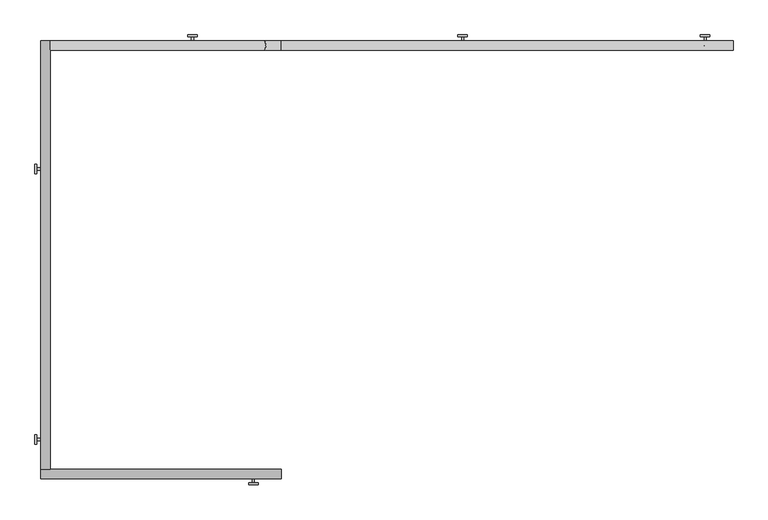
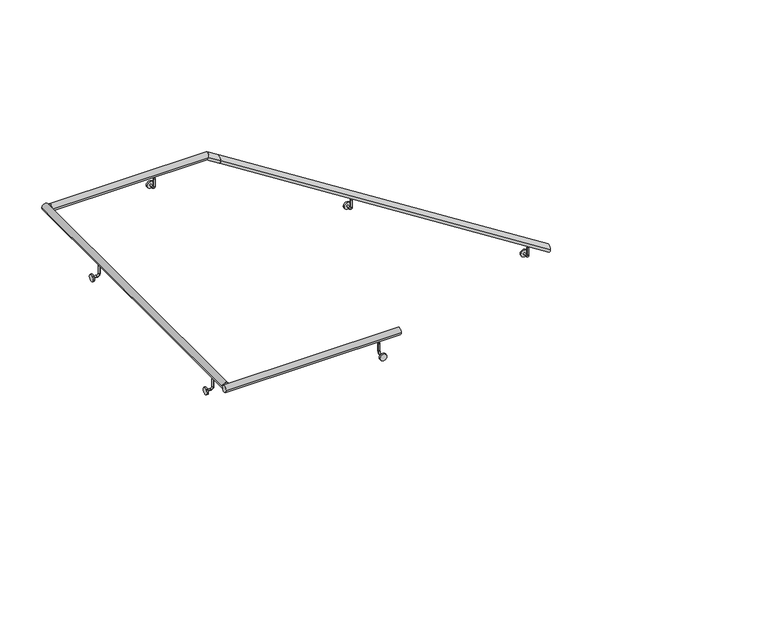
"""IFC4 building model written with IfcOpenShell, lengths in millimetres: railing geometry."""

from ifc_helpers import new_model, si_unit, point, frame, frame_2d, origin, place, context, project, spatial, circle_curve, ellipse_curve, trimmed, segment, composite_curve, outline, extrude, source, transform, mapped, element, save
from ifc_brep_helpers import plane_surface, cylinder_surface, revolved_surface, advanced_brep


def railing_d584f0b8(model_context):
    return source(origin(), model_context, "Body", "SolidModel", [
        advanced_brep(
        [(-47747.4858495, 17739.1574868, 4652.1467196), (-47747.4858495, 17789.1574868, 4652.1467196), (-50177.4858495, 17739.1574868, 6195.0038624), (-50177.4858495, 17789.1574868, 6195.0038624)],
        [
            (0, 1, ellipse_curve(frame((-47747.4858495, 17764.1574868, 4652.1467196), z_axis=(1.0, 0.0, 0.0), x_axis=(0.0, 0.0, -1.0)), 29.613386, 25.0)),
            (1, 0, ellipse_curve(frame((-47747.4858495, 17764.1574868, 4652.1467196), z_axis=(1.0, 0.0, 0.0), x_axis=(0.0, 0.0, -1.0)), 29.613386, 25.0)),
            (2, 3, ellipse_curve(frame((-50177.4858495, 17764.1574868, 6195.0038624), z_axis=(-1.0, 0.0, 0.0), x_axis=(0.0, 0.0, -1.0)), 29.613386, 25.0)),
            (3, 2, ellipse_curve(frame((-50177.4858495, 17764.1574868, 6195.0038624), z_axis=(-1.0, 0.0, 0.0), x_axis=(0.0, 0.0, -1.0)), 29.613386, 25.0)),
            (0, 2),
            (3, 1),
        ],
        [
            plane_surface(frame((-47747.4858495, 17764.1574868, 4681.7601056), z_axis=(1.0, 0.0, 0.0), x_axis=(0.0, -1.0, 0.0))),
            plane_surface(frame((-50177.4858495, 17764.1574868, 6224.6172485), z_axis=(-1.0, 0.0, 0.0), x_axis=(0.0, -1.0, 0.0))),
            cylinder_surface(frame((-47760.8860529, 17764.1574868, 4660.6547852), z_axis=(0.8442128152478047, 0.0, -0.5360081366652713), x_axis=(0.0, 1.0, 0.0)), 25.0),
        ],
        [
            (0, [[1, 2]]),
            (1, [[3, 4]]),
            (2, [[-1, 5, -4, 6]]),
            (2, [[-2, -6, -3, -5]]),
        ],
    ),
        advanced_brep(
        [(-50177.4858495, 17739.1574868, 6195.0038624), (-50177.4858495, 17789.1574868, 6195.0038624), (-50268.4797662, 17739.1574868, 6252.7777778), (-50268.4797662, 17789.1574868, 6252.7777778), (-51419.7848926, 17739.1574868, 6252.7777778), (-51419.7848926, 17789.1574868, 6252.7777778)],
        [
            (0, 1, ellipse_curve(frame((-50177.4858495, 17764.1574868, 6195.0038624), z_axis=(1.0, 0.0, 0.0), x_axis=(0.0, 0.0, -1.0)), 29.613386, 25.0)),
            (1, 0, ellipse_curve(frame((-50177.4858495, 17764.1574868, 6195.0038624), z_axis=(1.0, 0.0, 0.0), x_axis=(0.0, 0.0, -1.0)), 29.613386, 25.0)),
            (0, 2),
            (2, 3, ellipse_curve(frame((-50268.4797662, 17764.1574868, 6252.7777778), z_axis=(0.9602637177483601, 0.0, -0.27909423565544655), x_axis=(-0.2790942356554468, 0.0, -0.9602637177483601)), 26.0345148, 25.0)),
            (3, 1),
            (3, 2, ellipse_curve(frame((-50268.4797662, 17764.1574868, 6252.7777778), z_axis=(0.9602637177483601, 0.0, -0.27909423565544655), x_axis=(-0.2790942356554468, 0.0, -0.9602637177483601)), 26.0345148, 25.0)),
            (4, 5, circle_curve(frame((-51419.7848926, 17764.1574868, 6252.7777778), z_axis=(-1.0, 0.0, 0.0), x_axis=(0.0, 1.0, 0.0)), 25.0)),
            (5, 4, circle_curve(frame((-51419.7848926, 17764.1574868, 6252.7777778), z_axis=(-1.0, 0.0, 0.0), x_axis=(0.0, 1.0, 0.0)), 25.0)),
            (2, 4),
            (5, 3),
        ],
        [
            plane_surface(frame((-50177.4858495, 17764.1574868, 6224.6172485), z_axis=(1.0, 0.0, 0.0), x_axis=(0.0, -1.0, 0.0))),
            cylinder_surface(frame((-50190.8860529, 17764.1574868, 6203.5119281), z_axis=(0.844212815247804, 0.0, -0.5360081366652723), x_axis=(0.0, 1.0, 0.0)), 25.0),
            plane_surface(frame((-51419.7848926, 17764.1574868, 6277.7777778), z_axis=(-1.0, 0.0, 0.0), x_axis=(0.0, -1.0, 0.0))),
            cylinder_surface(frame((-50261.2136831, 17764.1574868, 6252.7777778), z_axis=(1.0, 0.0, 0.0), x_axis=(0.0, 1.0, 0.0)), 25.0),
        ],
        [
            (0, [[1, 2]]),
            (1, [[-1, 3, 4, 5]]),
            (1, [[-2, -5, 6, -3]]),
            (2, [[7, 8]]),
            (3, [[-4, 9, -8, 10]]),
            (3, [[-6, -10, -7, -9]]),
        ],
    ),
        advanced_brep(
        [(-51419.7848926, 17789.1574868, 6252.7777778), (-51469.7848926, 17789.1574868, 6252.7777778), (-51419.7848926, 15484.3574868, 6252.7777778), (-51469.7848926, 15484.3574868, 6252.7777778)],
        [
            (0, 1, circle_curve(frame((-51444.7848926, 17789.1574868, 6252.7777778), z_axis=(0.0, 1.0, 0.0), x_axis=(-1.0, 0.0, 0.0)), 25.0)),
            (1, 0, circle_curve(frame((-51444.7848926, 17789.1574868, 6252.7777778), z_axis=(0.0, 1.0, 0.0), x_axis=(-1.0, 0.0, 0.0)), 25.0)),
            (2, 3, circle_curve(frame((-51444.7848926, 15484.3574868, 6252.7777778), z_axis=(0.0, -1.0, 0.0), x_axis=(-1.0, 0.0, 0.0)), 25.0)),
            (3, 2, circle_curve(frame((-51444.7848926, 15484.3574868, 6252.7777778), z_axis=(0.0, -1.0, 0.0), x_axis=(-1.0, 0.0, 0.0)), 25.0)),
            (0, 2),
            (3, 1),
        ],
        [
            plane_surface(frame((-51444.7848926, 17789.1574868, 6277.7777778), z_axis=(0.0, 1.0, 0.0), x_axis=(0.0, 0.0, -1.0))),
            plane_surface(frame((-51444.7848926, 15484.3574868, 6277.7777778), z_axis=(0.0, -1.0, 0.0), x_axis=(0.0, 0.0, -1.0))),
            cylinder_surface(frame((-51444.7848926, 17789.1574868, 6252.7777778), z_axis=(0.0, 1.0, 0.0), x_axis=(-1.0, 0.0, 0.0)), 25.0),
        ],
        [
            (0, [[1, 2]]),
            (1, [[3, 4]]),
            (2, [[-1, 5, -4, 6]]),
            (2, [[-2, -6, -3, -5]]),
        ],
    ),
        advanced_brep(
        [(-51469.7848926, 15484.3574868, 6252.7777778), (-51469.7848926, 15434.3574868, 6252.7777778), (-50177.4858495, 15484.3574868, 6252.7777778), (-50177.4858495, 15434.3574868, 6252.7777778)],
        [
            (0, 1, circle_curve(frame((-51469.7848926, 15459.3574868, 6252.7777778), z_axis=(-1.0, 0.0, 0.0), x_axis=(0.0, -1.0, 0.0)), 25.0)),
            (1, 0, circle_curve(frame((-51469.7848926, 15459.3574868, 6252.7777778), z_axis=(-1.0, 0.0, 0.0), x_axis=(0.0, -1.0, 0.0)), 25.0)),
            (2, 3, circle_curve(frame((-50177.4858495, 15459.3574868, 6252.7777778), z_axis=(1.0, 0.0, 0.0), x_axis=(0.0, -1.0, 0.0)), 25.0)),
            (3, 2, circle_curve(frame((-50177.4858495, 15459.3574868, 6252.7777778), z_axis=(1.0, 0.0, 0.0), x_axis=(0.0, -1.0, 0.0)), 25.0)),
            (0, 2),
            (3, 1),
        ],
        [
            plane_surface(frame((-51469.7848926, 15459.3574868, 6277.7777778), z_axis=(-1.0, 0.0, 0.0), x_axis=(0.0, 1.0, 0.0))),
            plane_surface(frame((-50177.4858495, 15459.3574868, 6277.7777778), z_axis=(1.0, 0.0, 0.0), x_axis=(0.0, 1.0, 0.0))),
            cylinder_surface(frame((-51469.7848926, 15459.3574868, 6252.7777778), z_axis=(-1.0, 0.0, 0.0), x_axis=(0.0, -1.0, 0.0)), 25.0),
        ],
        [
            (0, [[1, 2]]),
            (1, [[3, 4]]),
            (2, [[-1, 5, -4, 6]]),
            (2, [[-2, -6, -3, -5]]),
        ],
    ),
        advanced_brep(
        [(-51444.7848926, 15652.288061, 6208.7277778), (-51444.7848926, 15639.588061, 6208.7277778), (-51444.7848926, 15652.288061, 6151.5777778), (-51444.7848926, 15639.588061, 6151.5777778), (-51463.8348926, 15639.588061, 6132.5277778), (-51463.8348926, 15652.288061, 6132.5277778), (-51492.4098926, 15652.288061, 6132.5277778), (-51492.4098926, 15639.588061, 6132.5277778)],
        [
            (0, 1, circle_curve(frame((-51444.7848926, 15645.938061, 6208.7277778), z_axis=(0.0, 0.0, 1.0), x_axis=(0.0, -1.0, 0.0)), 6.35)),
            (1, 0, circle_curve(frame((-51444.7848926, 15645.938061, 6208.7277778), z_axis=(0.0, 0.0, 1.0), x_axis=(0.0, -1.0, 0.0)), 6.35)),
            (0, 2),
            (2, 3, circle_curve(frame((-51444.7848926, 15645.938061, 6151.5777778), z_axis=(0.0, 0.0, 1.0), x_axis=(0.0, -1.0, 0.0)), 6.35)),
            (3, 1),
            (3, 2, circle_curve(frame((-51444.7848926, 15645.938061, 6151.5777778), z_axis=(0.0, 0.0, 1.0), x_axis=(0.0, -1.0, 0.0)), 6.35)),
            (4, 3, circle_curve(frame((-51463.8348926, 15639.588061, 6151.5777778), z_axis=(0.0, -1.0, 0.0), x_axis=(1.0, 0.0, 0.0)), 19.05)),
            (2, 5, circle_curve(frame((-51463.8348926, 15652.288061, 6151.5777778), z_axis=(0.0, 1.0, 0.0), x_axis=(1.0, 0.0, 0.0)), 19.05)),
            (5, 4, circle_curve(frame((-51463.8348926, 15645.938061, 6132.5277778), z_axis=(1.0, 0.0, 0.0), x_axis=(0.0, -1.0, 0.0)), 6.35)),
            (4, 5, circle_curve(frame((-51463.8348926, 15645.938061, 6132.5277778), z_axis=(1.0, 0.0, 0.0), x_axis=(0.0, -1.0, 0.0)), 6.35)),
            (6, 7, circle_curve(frame((-51492.4098926, 15645.938061, 6132.5277778), z_axis=(-1.0, 0.0, 0.0), x_axis=(0.0, -1.0, 0.0)), 6.35)),
            (7, 6, circle_curve(frame((-51492.4098926, 15645.938061, 6132.5277778), z_axis=(-1.0, 0.0, 0.0), x_axis=(0.0, -1.0, 0.0)), 6.35)),
            (5, 6),
            (7, 4),
        ],
        [
            plane_surface(frame((-51444.7848926, 15639.588061, 6208.7277778), z_axis=(0.0, 0.0, 1.0), x_axis=(-1.0, 0.0, 0.0))),
            cylinder_surface(frame((-51444.7848926, 15645.938061, 6208.7277778), z_axis=(0.0, 0.0, 1.0), x_axis=(0.0, -1.0, 0.0)), 6.35),
            revolved_surface(trimmed(ellipse_curve(frame((-51444.7848926, 15645.938061, 6151.5777778), z_axis=(0.0, 0.0, 1.0), x_axis=(0.0, -1.0, 0.0)), 6.35, 6.35), [point((-51444.7848926, 15652.288061, 6151.5777778))], [point((-51444.7848926, 15639.588061, 6151.5777778))], True, "CARTESIAN"), (-51463.8348926, 15645.938061, 6151.5777778), (0.0, 1.0, 0.0)),
            revolved_surface(trimmed(ellipse_curve(frame((-51444.7848926, 15645.938061, 6151.5777778), z_axis=(0.0, 0.0, 1.0), x_axis=(0.0, -1.0, 0.0)), 6.35, 6.35), [point((-51444.7848926, 15639.588061, 6151.5777778))], [point((-51444.7848926, 15652.288061, 6151.5777778))], True, "CARTESIAN"), (-51463.8348926, 15645.938061, 6151.5777778), (0.0, 1.0, 0.0)),
            plane_surface(frame((-51492.4098926, 15645.938061, 6126.1777778), z_axis=(-1.0, 0.0, 0.0), x_axis=(0.0, -1.0, 0.0))),
            cylinder_surface(frame((-51463.8348926, 15645.938061, 6132.5277778), z_axis=(1.0, 0.0, 0.0), x_axis=(0.0, -1.0, 0.0)), 6.35),
        ],
        [
            (0, [[1, 2]]),
            (1, [[-1, 3, 4, 5]]),
            (1, [[-2, -5, 6, -3]]),
            (2, [[7, -4, 8, 9]]),
            (3, [[-8, -6, -7, 10]]),
            (4, [[11, 12]]),
            (5, [[-9, 13, -12, 14]]),
            (5, [[-10, -14, -11, -13]]),
        ],
    ),
        extrude(outline(composite_curve([segment(trimmed(circle_curve(frame_2d((15645.938061, 6132.5277778)), 25.4), [point((15620.538061, 6132.5277778))], [point((15671.338061, 6132.5277778))], False, "CARTESIAN"), True, "CONTINUOUS"), segment(trimmed(circle_curve(frame_2d((15645.938061, 6132.5277778)), 25.4), [point((15671.338061, 6132.5277778))], [point((15620.538061, 6132.5277778))], False, "CARTESIAN"), True, "CONTINUOUS")], self_intersect=False)), frame((-51501.9348926, 0.0, 0.0), z_axis=(1.0, 0.0, 0.0), x_axis=(0.0, 1.0, 0.0)), (0.0, 0.0, 1.0), 9.525),
        advanced_brep(
        [(-51444.7848926, 17106.1676782, 6208.7277778), (-51444.7848926, 17093.4676782, 6208.7277778), (-51444.7848926, 17106.1676782, 6151.5777778), (-51444.7848926, 17093.4676782, 6151.5777778), (-51463.8348926, 17093.4676782, 6132.5277778), (-51463.8348926, 17106.1676782, 6132.5277778), (-51492.4098926, 17106.1676782, 6132.5277778), (-51492.4098926, 17093.4676782, 6132.5277778)],
        [
            (0, 1, circle_curve(frame((-51444.7848926, 17099.8176782, 6208.7277778), z_axis=(0.0, 0.0, 1.0), x_axis=(0.0, -1.0, 0.0)), 6.35)),
            (1, 0, circle_curve(frame((-51444.7848926, 17099.8176782, 6208.7277778), z_axis=(0.0, 0.0, 1.0), x_axis=(0.0, -1.0, 0.0)), 6.35)),
            (0, 2),
            (2, 3, circle_curve(frame((-51444.7848926, 17099.8176782, 6151.5777778), z_axis=(0.0, 0.0, 1.0), x_axis=(0.0, -1.0, 0.0)), 6.35)),
            (3, 1),
            (3, 2, circle_curve(frame((-51444.7848926, 17099.8176782, 6151.5777778), z_axis=(0.0, 0.0, 1.0), x_axis=(0.0, -1.0, 0.0)), 6.35)),
            (4, 3, circle_curve(frame((-51463.8348926, 17093.4676782, 6151.5777778), z_axis=(0.0, -1.0, 0.0), x_axis=(1.0, 0.0, 0.0)), 19.05)),
            (2, 5, circle_curve(frame((-51463.8348926, 17106.1676782, 6151.5777778), z_axis=(0.0, 1.0, 0.0), x_axis=(1.0, 0.0, 0.0)), 19.05)),
            (5, 4, circle_curve(frame((-51463.8348926, 17099.8176782, 6132.5277778), z_axis=(1.0, 0.0, 0.0), x_axis=(0.0, -1.0, 0.0)), 6.35)),
            (4, 5, circle_curve(frame((-51463.8348926, 17099.8176782, 6132.5277778), z_axis=(1.0, 0.0, 0.0), x_axis=(0.0, -1.0, 0.0)), 6.35)),
            (6, 7, circle_curve(frame((-51492.4098926, 17099.8176782, 6132.5277778), z_axis=(-1.0, 0.0, 0.0), x_axis=(0.0, -1.0, 0.0)), 6.35)),
            (7, 6, circle_curve(frame((-51492.4098926, 17099.8176782, 6132.5277778), z_axis=(-1.0, 0.0, 0.0), x_axis=(0.0, -1.0, 0.0)), 6.35)),
            (5, 6),
            (7, 4),
        ],
        [
            plane_surface(frame((-51444.7848926, 17093.4676782, 6208.7277778), z_axis=(0.0, 0.0, 1.0), x_axis=(-1.0, 0.0, 0.0))),
            cylinder_surface(frame((-51444.7848926, 17099.8176782, 6208.7277778), z_axis=(0.0, 0.0, 1.0), x_axis=(0.0, -1.0, 0.0)), 6.35),
            revolved_surface(trimmed(ellipse_curve(frame((-51444.7848926, 17099.8176782, 6151.5777778), z_axis=(0.0, 0.0, 1.0), x_axis=(0.0, -1.0, 0.0)), 6.35, 6.35), [point((-51444.7848926, 17106.1676782, 6151.5777778))], [point((-51444.7848926, 17093.4676782, 6151.5777778))], True, "CARTESIAN"), (-51463.8348926, 17099.8176782, 6151.5777778), (0.0, 1.0, 0.0)),
            revolved_surface(trimmed(ellipse_curve(frame((-51444.7848926, 17099.8176782, 6151.5777778), z_axis=(0.0, 0.0, 1.0), x_axis=(0.0, -1.0, 0.0)), 6.35, 6.35), [point((-51444.7848926, 17093.4676782, 6151.5777778))], [point((-51444.7848926, 17106.1676782, 6151.5777778))], True, "CARTESIAN"), (-51463.8348926, 17099.8176782, 6151.5777778), (0.0, 1.0, 0.0)),
            plane_surface(frame((-51492.4098926, 17099.8176782, 6126.1777778), z_axis=(-1.0, 0.0, 0.0), x_axis=(0.0, -1.0, 0.0))),
            cylinder_surface(frame((-51463.8348926, 17099.8176782, 6132.5277778), z_axis=(1.0, 0.0, 0.0), x_axis=(0.0, -1.0, 0.0)), 6.35),
        ],
        [
            (0, [[1, 2]]),
            (1, [[-1, 3, 4, 5]]),
            (1, [[-2, -5, 6, -3]]),
            (2, [[7, -4, 8, 9]]),
            (3, [[-8, -6, -7, 10]]),
            (4, [[11, 12]]),
            (5, [[-9, 13, -12, 14]]),
            (5, [[-10, -14, -11, -13]]),
        ],
    ),
        extrude(outline(composite_curve([segment(trimmed(circle_curve(frame_2d((17099.8176782, 6132.5277778)), 25.4), [point((17074.4176782, 6132.5277778))], [point((17125.2176782, 6132.5277778))], False, "CARTESIAN"), True, "CONTINUOUS"), segment(trimmed(circle_curve(frame_2d((17099.8176782, 6132.5277778)), 25.4), [point((17125.2176782, 6132.5277778))], [point((17074.4176782, 6132.5277778))], False, "CARTESIAN"), True, "CONTINUOUS")], self_intersect=False)), frame((-51501.9348926, 0.0, 0.0), z_axis=(1.0, 0.0, 0.0), x_axis=(0.0, 1.0, 0.0)), (0.0, 0.0, 1.0), 9.525),
        advanced_brep(
        [(-50648.895084, 17764.1574868, 6208.7277778), (-50661.595084, 17764.1574868, 6208.7277778), (-50648.895084, 17764.1574868, 6151.5777778), (-50661.595084, 17764.1574868, 6151.5777778), (-50661.595084, 17783.2074868, 6132.5277778), (-50648.895084, 17783.2074868, 6132.5277778), (-50648.895084, 17811.7824868, 6132.5277778), (-50661.595084, 17811.7824868, 6132.5277778)],
        [
            (0, 1, circle_curve(frame((-50655.245084, 17764.1574868, 6208.7277778), z_axis=(0.0, 0.0, 1.0), x_axis=(-1.0, 0.0, 0.0)), 6.35)),
            (1, 0, circle_curve(frame((-50655.245084, 17764.1574868, 6208.7277778), z_axis=(0.0, 0.0, 1.0), x_axis=(-1.0, 0.0, 0.0)), 6.35)),
            (0, 2),
            (2, 3, circle_curve(frame((-50655.245084, 17764.1574868, 6151.5777778), z_axis=(0.0, 0.0, 1.0), x_axis=(-1.0, 0.0, 0.0)), 6.35)),
            (3, 1),
            (3, 2, circle_curve(frame((-50655.245084, 17764.1574868, 6151.5777778), z_axis=(0.0, 0.0, 1.0), x_axis=(-1.0, 0.0, 0.0)), 6.35)),
            (4, 3, circle_curve(frame((-50661.595084, 17783.2074868, 6151.5777778), z_axis=(-1.0, 0.0, 0.0), x_axis=(0.0, -1.0, 0.0)), 19.05)),
            (2, 5, circle_curve(frame((-50648.895084, 17783.2074868, 6151.5777778), z_axis=(1.0, 0.0, 0.0), x_axis=(0.0, -1.0, 0.0)), 19.05)),
            (5, 4, circle_curve(frame((-50655.245084, 17783.2074868, 6132.5277778), z_axis=(0.0, -1.0, 0.0), x_axis=(-1.0, 0.0, 0.0)), 6.35)),
            (4, 5, circle_curve(frame((-50655.245084, 17783.2074868, 6132.5277778), z_axis=(0.0, -1.0, 0.0), x_axis=(-1.0, 0.0, 0.0)), 6.35)),
            (6, 7, circle_curve(frame((-50655.245084, 17811.7824868, 6132.5277778), z_axis=(0.0, 1.0, 0.0), x_axis=(-1.0, 0.0, 0.0)), 6.35)),
            (7, 6, circle_curve(frame((-50655.245084, 17811.7824868, 6132.5277778), z_axis=(0.0, 1.0, 0.0), x_axis=(-1.0, 0.0, 0.0)), 6.35)),
            (5, 6),
            (7, 4),
        ],
        [
            plane_surface(frame((-50661.595084, 17764.1574868, 6208.7277778), z_axis=(0.0, 0.0, 1.0), x_axis=(0.0, 1.0, 0.0))),
            cylinder_surface(frame((-50655.245084, 17764.1574868, 6208.7277778), z_axis=(0.0, 0.0, 1.0), x_axis=(-1.0, 0.0, 0.0)), 6.35),
            revolved_surface(trimmed(ellipse_curve(frame((-50655.245084, 17764.1574868, 6151.5777778), z_axis=(0.0, 0.0, 1.0), x_axis=(-1.0, 0.0, 0.0)), 6.35, 6.35), [point((-50648.895084, 17764.1574868, 6151.5777778))], [point((-50661.595084, 17764.1574868, 6151.5777778))], True, "CARTESIAN"), (-50655.245084, 17783.2074868, 6151.5777778), (1.0, 0.0, 0.0)),
            revolved_surface(trimmed(ellipse_curve(frame((-50655.245084, 17764.1574868, 6151.5777778), z_axis=(0.0, 0.0, 1.0), x_axis=(-1.0, 0.0, 0.0)), 6.35, 6.35), [point((-50661.595084, 17764.1574868, 6151.5777778))], [point((-50648.895084, 17764.1574868, 6151.5777778))], True, "CARTESIAN"), (-50655.245084, 17783.2074868, 6151.5777778), (1.0, 0.0, 0.0)),
            plane_surface(frame((-50655.245084, 17811.7824868, 6126.1777778), z_axis=(0.0, 1.0, 0.0), x_axis=(-1.0, 0.0, 0.0))),
            cylinder_surface(frame((-50655.245084, 17783.2074868, 6132.5277778), z_axis=(0.0, -1.0, 0.0), x_axis=(-1.0, 0.0, 0.0)), 6.35),
        ],
        [
            (0, [[1, 2]]),
            (1, [[-1, 3, 4, 5]]),
            (1, [[-2, -5, 6, -3]]),
            (2, [[7, -4, 8, 9]]),
            (3, [[-8, -6, -7, 10]]),
            (4, [[11, 12]]),
            (5, [[-9, 13, -12, 14]]),
            (5, [[-10, -14, -11, -13]]),
        ],
    ),
        extrude(outline(composite_curve([segment(trimmed(circle_curve(frame_2d((6132.5277778, -50655.245084)), 25.4), [point((6132.5277778, -50680.645084))], [point((6132.5277778, -50629.845084))], False, "CARTESIAN"), True, "CONTINUOUS"), segment(trimmed(circle_curve(frame_2d((6132.5277778, -50655.245084)), 25.4), [point((6132.5277778, -50629.845084))], [point((6132.5277778, -50680.645084))], False, "CARTESIAN"), True, "CONTINUOUS")], self_intersect=False)), frame((0.0, 17811.7824868, 0.0), z_axis=(0.0, 1.0, 0.0), x_axis=(0.0, 0.0, 1.0)), (0.0, 0.0, 1.0), 9.525),
        advanced_brep(
        [(-49195.0154667, 17764.1574868, 5535.8082753), (-49207.7154667, 17764.1574868, 5535.8082753), (-49195.0154667, 17764.1574868, 5478.6582753), (-49207.7154667, 17764.1574868, 5478.6582753), (-49207.7154667, 17783.2074868, 5459.6082753), (-49195.0154667, 17783.2074868, 5459.6082753), (-49195.0154667, 17811.7824868, 5459.6082753), (-49207.7154667, 17811.7824868, 5459.6082753)],
        [
            (0, 1, circle_curve(frame((-49201.3654667, 17764.1574868, 5535.8082753), z_axis=(0.0, 0.0, 1.0), x_axis=(-1.0, 0.0, 0.0)), 6.35)),
            (1, 0, circle_curve(frame((-49201.3654667, 17764.1574868, 5535.8082753), z_axis=(0.0, 0.0, 1.0), x_axis=(-1.0, 0.0, 0.0)), 6.35)),
            (0, 2),
            (2, 3, circle_curve(frame((-49201.3654667, 17764.1574868, 5478.6582753), z_axis=(0.0, 0.0, 1.0), x_axis=(-1.0, 0.0, 0.0)), 6.35)),
            (3, 1),
            (3, 2, circle_curve(frame((-49201.3654667, 17764.1574868, 5478.6582753), z_axis=(0.0, 0.0, 1.0), x_axis=(-1.0, 0.0, 0.0)), 6.35)),
            (4, 3, circle_curve(frame((-49207.7154667, 17783.2074868, 5478.6582753), z_axis=(-1.0, 0.0, 0.0), x_axis=(0.0, -1.0, 0.0)), 19.05)),
            (2, 5, circle_curve(frame((-49195.0154667, 17783.2074868, 5478.6582753), z_axis=(1.0, 0.0, 0.0), x_axis=(0.0, -1.0, 0.0)), 19.05)),
            (5, 4, circle_curve(frame((-49201.3654667, 17783.2074868, 5459.6082753), z_axis=(0.0, -1.0, 0.0), x_axis=(-1.0, 0.0, 0.0)), 6.35)),
            (4, 5, circle_curve(frame((-49201.3654667, 17783.2074868, 5459.6082753), z_axis=(0.0, -1.0, 0.0), x_axis=(-1.0, 0.0, 0.0)), 6.35)),
            (6, 7, circle_curve(frame((-49201.3654667, 17811.7824868, 5459.6082753), z_axis=(0.0, 1.0, 0.0), x_axis=(-1.0, 0.0, 0.0)), 6.35)),
            (7, 6, circle_curve(frame((-49201.3654667, 17811.7824868, 5459.6082753), z_axis=(0.0, 1.0, 0.0), x_axis=(-1.0, 0.0, 0.0)), 6.35)),
            (5, 6),
            (7, 4),
        ],
        [
            plane_surface(frame((-49207.7154667, 17764.1574868, 5535.8082753), z_axis=(0.0, 0.0, 1.0), x_axis=(0.0, 1.0, 0.0))),
            cylinder_surface(frame((-49201.3654667, 17764.1574868, 5535.8082753), z_axis=(0.0, 0.0, 1.0), x_axis=(-1.0, 0.0, 0.0)), 6.35),
            revolved_surface(trimmed(ellipse_curve(frame((-49201.3654667, 17764.1574868, 5478.6582753), z_axis=(0.0, 0.0, 1.0), x_axis=(-1.0, 0.0, 0.0)), 6.35, 6.35), [point((-49195.0154667, 17764.1574868, 5478.6582753))], [point((-49207.7154667, 17764.1574868, 5478.6582753))], True, "CARTESIAN"), (-49201.3654667, 17783.2074868, 5478.6582753), (1.0, 0.0, 0.0)),
            revolved_surface(trimmed(ellipse_curve(frame((-49201.3654667, 17764.1574868, 5478.6582753), z_axis=(0.0, 0.0, 1.0), x_axis=(-1.0, 0.0, 0.0)), 6.35, 6.35), [point((-49207.7154667, 17764.1574868, 5478.6582753))], [point((-49195.0154667, 17764.1574868, 5478.6582753))], True, "CARTESIAN"), (-49201.3654667, 17783.2074868, 5478.6582753), (1.0, 0.0, 0.0)),
            plane_surface(frame((-49201.3654667, 17811.7824868, 5453.2582753), z_axis=(0.0, 1.0, 0.0), x_axis=(-1.0, 0.0, 0.0))),
            cylinder_surface(frame((-49201.3654667, 17783.2074868, 5459.6082753), z_axis=(0.0, -1.0, 0.0), x_axis=(-1.0, 0.0, 0.0)), 6.35),
        ],
        [
            (0, [[1, 2]]),
            (1, [[-1, 3, 4, 5]]),
            (1, [[-2, -5, 6, -3]]),
            (2, [[7, -4, 8, 9]]),
            (3, [[-8, -6, -7, 10]]),
            (4, [[11, 12]]),
            (5, [[-9, 13, -12, 14]]),
            (5, [[-10, -14, -11, -13]]),
        ],
    ),
        extrude(outline(composite_curve([segment(trimmed(circle_curve(frame_2d((5459.6082753, -49201.3654667)), 25.4), [point((5459.6082753, -49226.7654667))], [point((5459.6082753, -49175.9654667))], False, "CARTESIAN"), True, "CONTINUOUS"), segment(trimmed(circle_curve(frame_2d((5459.6082753, -49201.3654667)), 25.4), [point((5459.6082753, -49175.9654667))], [point((5459.6082753, -49226.7654667))], False, "CARTESIAN"), True, "CONTINUOUS")], self_intersect=False)), frame((0.0, 17811.7824868, 0.0), z_axis=(0.0, 1.0, 0.0), x_axis=(0.0, 0.0, 1.0)), (0.0, 0.0, 1.0), 9.525),
        advanced_brep(
        [(-50333.8358495, 15459.3574868, 6208.7277778), (-50321.1358495, 15459.3574868, 6208.7277778), (-50333.8358495, 15459.3574868, 6151.5777778), (-50321.1358495, 15459.3574868, 6151.5777778), (-50321.1358495, 15440.3074868, 6132.5277778), (-50333.8358495, 15440.3074868, 6132.5277778), (-50333.8358495, 15411.7324868, 6132.5277778), (-50321.1358495, 15411.7324868, 6132.5277778)],
        [
            (0, 1, circle_curve(frame((-50327.4858495, 15459.3574868, 6208.7277778), z_axis=(0.0, 0.0, 1.0), x_axis=(1.0, 0.0, 0.0)), 6.35)),
            (1, 0, circle_curve(frame((-50327.4858495, 15459.3574868, 6208.7277778), z_axis=(0.0, 0.0, 1.0), x_axis=(1.0, 0.0, 0.0)), 6.35)),
            (0, 2),
            (2, 3, circle_curve(frame((-50327.4858495, 15459.3574868, 6151.5777778), z_axis=(0.0, 0.0, 1.0), x_axis=(1.0, 0.0, 0.0)), 6.35)),
            (3, 1),
            (3, 2, circle_curve(frame((-50327.4858495, 15459.3574868, 6151.5777778), z_axis=(0.0, 0.0, 1.0), x_axis=(1.0, 0.0, 0.0)), 6.35)),
            (4, 3, circle_curve(frame((-50321.1358495, 15440.3074868, 6151.5777778), z_axis=(1.0, 0.0, 0.0), x_axis=(0.0, 1.0, 0.0)), 19.05)),
            (2, 5, circle_curve(frame((-50333.8358495, 15440.3074868, 6151.5777778), z_axis=(-1.0, 0.0, 0.0), x_axis=(0.0, 1.0, 0.0)), 19.05)),
            (5, 4, circle_curve(frame((-50327.4858495, 15440.3074868, 6132.5277778), z_axis=(0.0, 1.0, 0.0), x_axis=(1.0, 0.0, 0.0)), 6.35)),
            (4, 5, circle_curve(frame((-50327.4858495, 15440.3074868, 6132.5277778), z_axis=(0.0, 1.0, 0.0), x_axis=(1.0, 0.0, 0.0)), 6.35)),
            (6, 7, circle_curve(frame((-50327.4858495, 15411.7324868, 6132.5277778), z_axis=(0.0, -1.0, 0.0), x_axis=(1.0, 0.0, 0.0)), 6.35)),
            (7, 6, circle_curve(frame((-50327.4858495, 15411.7324868, 6132.5277778), z_axis=(0.0, -1.0, 0.0), x_axis=(1.0, 0.0, 0.0)), 6.35)),
            (5, 6),
            (7, 4),
        ],
        [
            plane_surface(frame((-50321.1358495, 15459.3574868, 6208.7277778), z_axis=(0.0, 0.0, 1.0), x_axis=(0.0, -1.0, 0.0))),
            cylinder_surface(frame((-50327.4858495, 15459.3574868, 6208.7277778), z_axis=(0.0, 0.0, 1.0), x_axis=(1.0, 0.0, 0.0)), 6.35),
            revolved_surface(trimmed(ellipse_curve(frame((-50327.4858495, 15459.3574868, 6151.5777778), z_axis=(0.0, 0.0, 1.0), x_axis=(1.0, 0.0, 0.0)), 6.35, 6.35), [point((-50333.8358495, 15459.3574868, 6151.5777778))], [point((-50321.1358495, 15459.3574868, 6151.5777778))], True, "CARTESIAN"), (-50327.4858495, 15440.3074868, 6151.5777778), (-1.0, 0.0, 0.0)),
            revolved_surface(trimmed(ellipse_curve(frame((-50327.4858495, 15459.3574868, 6151.5777778), z_axis=(0.0, 0.0, 1.0), x_axis=(1.0, 0.0, 0.0)), 6.35, 6.35), [point((-50321.1358495, 15459.3574868, 6151.5777778))], [point((-50333.8358495, 15459.3574868, 6151.5777778))], True, "CARTESIAN"), (-50327.4858495, 15440.3074868, 6151.5777778), (-1.0, 0.0, 0.0)),
            plane_surface(frame((-50327.4858495, 15411.7324868, 6126.1777778), z_axis=(0.0, -1.0, 0.0), x_axis=(1.0, 0.0, 0.0))),
            cylinder_surface(frame((-50327.4858495, 15440.3074868, 6132.5277778), z_axis=(0.0, 1.0, 0.0), x_axis=(1.0, 0.0, 0.0)), 6.35),
        ],
        [
            (0, [[1, 2]]),
            (1, [[-1, 3, 4, 5]]),
            (1, [[-2, -5, 6, -3]]),
            (2, [[7, -4, 8, 9]]),
            (3, [[-8, -6, -7, 10]]),
            (4, [[11, 12]]),
            (5, [[-9, 13, -12, 14]]),
            (5, [[-10, -14, -11, -13]]),
        ],
    ),
        extrude(outline(composite_curve([segment(trimmed(circle_curve(frame_2d((6132.5277778, -50327.4858495)), 25.4), [point((6132.5277778, -50302.0858495))], [point((6132.5277778, -50352.8858495))], False, "CARTESIAN"), True, "CONTINUOUS"), segment(trimmed(circle_curve(frame_2d((6132.5277778, -50327.4858495)), 25.4), [point((6132.5277778, -50352.8858495))], [point((6132.5277778, -50302.0858495))], False, "CARTESIAN"), True, "CONTINUOUS")], self_intersect=False)), frame((0.0, 15402.2074868, 0.0), z_axis=(0.0, 1.0, 0.0), x_axis=(0.0, 0.0, 1.0)), (0.0, 0.0, 1.0), 9.525),
        advanced_brep(
        [(-47891.1358495, 17764.1574868, 4707.9482009), (-47903.8358495, 17764.1574868, 4707.9482009), (-47891.1358495, 17764.1574868, 4650.7982009), (-47903.8358495, 17764.1574868, 4650.7982009), (-47903.8358495, 17783.2074868, 4631.7482009), (-47891.1358495, 17783.2074868, 4631.7482009), (-47891.1358495, 17811.7824868, 4631.7482009), (-47903.8358495, 17811.7824868, 4631.7482009)],
        [
            (0, 1, circle_curve(frame((-47897.4858495, 17764.1574868, 4707.9482009), z_axis=(0.0, 0.0, 1.0), x_axis=(-1.0, 0.0, 0.0)), 6.35)),
            (1, 0, circle_curve(frame((-47897.4858495, 17764.1574868, 4707.9482009), z_axis=(0.0, 0.0, 1.0), x_axis=(-1.0, 0.0, 0.0)), 6.35)),
            (0, 2),
            (2, 3, circle_curve(frame((-47897.4858495, 17764.1574868, 4650.7982009), z_axis=(0.0, 0.0, 1.0), x_axis=(-1.0, 0.0, 0.0)), 6.35)),
            (3, 1),
            (3, 2, circle_curve(frame((-47897.4858495, 17764.1574868, 4650.7982009), z_axis=(0.0, 0.0, 1.0), x_axis=(-1.0, 0.0, 0.0)), 6.35)),
            (4, 3, circle_curve(frame((-47903.8358495, 17783.2074868, 4650.7982009), z_axis=(-1.0, 0.0, 0.0), x_axis=(0.0, -1.0, 0.0)), 19.05)),
            (2, 5, circle_curve(frame((-47891.1358495, 17783.2074868, 4650.7982009), z_axis=(1.0, 0.0, 0.0), x_axis=(0.0, -1.0, 0.0)), 19.05)),
            (5, 4, circle_curve(frame((-47897.4858495, 17783.2074868, 4631.7482009), z_axis=(0.0, -1.0, 0.0), x_axis=(-1.0, 0.0, 0.0)), 6.35)),
            (4, 5, circle_curve(frame((-47897.4858495, 17783.2074868, 4631.7482009), z_axis=(0.0, -1.0, 0.0), x_axis=(-1.0, 0.0, 0.0)), 6.35)),
            (6, 7, circle_curve(frame((-47897.4858495, 17811.7824868, 4631.7482009), z_axis=(0.0, 1.0, 0.0), x_axis=(-1.0, 0.0, 0.0)), 6.35)),
            (7, 6, circle_curve(frame((-47897.4858495, 17811.7824868, 4631.7482009), z_axis=(0.0, 1.0, 0.0), x_axis=(-1.0, 0.0, 0.0)), 6.35)),
            (5, 6),
            (7, 4),
        ],
        [
            plane_surface(frame((-47903.8358495, 17764.1574868, 4707.9482009), z_axis=(0.0, 0.0, 1.0), x_axis=(0.0, 1.0, 0.0))),
            cylinder_surface(frame((-47897.4858495, 17764.1574868, 4707.9482009), z_axis=(0.0, 0.0, 1.0), x_axis=(-1.0, 0.0, 0.0)), 6.35),
            revolved_surface(trimmed(ellipse_curve(frame((-47897.4858495, 17764.1574868, 4650.7982009), z_axis=(0.0, 0.0, 1.0), x_axis=(-1.0, 0.0, 0.0)), 6.35, 6.35), [point((-47891.1358495, 17764.1574868, 4650.7982009))], [point((-47903.8358495, 17764.1574868, 4650.7982009))], True, "CARTESIAN"), (-47897.4858495, 17783.2074868, 4650.7982009), (1.0, 0.0, 0.0)),
            revolved_surface(trimmed(ellipse_curve(frame((-47897.4858495, 17764.1574868, 4650.7982009), z_axis=(0.0, 0.0, 1.0), x_axis=(-1.0, 0.0, 0.0)), 6.35, 6.35), [point((-47903.8358495, 17764.1574868, 4650.7982009))], [point((-47891.1358495, 17764.1574868, 4650.7982009))], True, "CARTESIAN"), (-47897.4858495, 17783.2074868, 4650.7982009), (1.0, 0.0, 0.0)),
            plane_surface(frame((-47897.4858495, 17811.7824868, 4625.3982009), z_axis=(0.0, 1.0, 0.0), x_axis=(-1.0, 0.0, 0.0))),
            cylinder_surface(frame((-47897.4858495, 17783.2074868, 4631.7482009), z_axis=(0.0, -1.0, 0.0), x_axis=(-1.0, 0.0, 0.0)), 6.35),
        ],
        [
            (0, [[1, 2]]),
            (1, [[-1, 3, 4, 5]]),
            (1, [[-2, -5, 6, -3]]),
            (2, [[7, -4, 8, 9]]),
            (3, [[-8, -6, -7, 10]]),
            (4, [[11, 12]]),
            (5, [[-9, 13, -12, 14]]),
            (5, [[-10, -14, -11, -13]]),
        ],
    ),
        extrude(outline(composite_curve([segment(trimmed(circle_curve(frame_2d((4631.7482009, -47897.4858495)), 25.4), [point((4631.7482009, -47922.8858495))], [point((4631.7482009, -47872.0858495))], False, "CARTESIAN"), True, "CONTINUOUS"), segment(trimmed(circle_curve(frame_2d((4631.7482009, -47897.4858495)), 25.4), [point((4631.7482009, -47872.0858495))], [point((4631.7482009, -47922.8858495))], False, "CARTESIAN"), True, "CONTINUOUS")], self_intersect=False)), frame((0.0, 17811.7824868, 0.0), z_axis=(0.0, 1.0, 0.0), x_axis=(0.0, 0.0, 1.0)), (0.0, 0.0, 1.0), 9.525),
    ])


if __name__ == "__main__":
    model = new_model("IFC4")
    model_context = context("Model", 3, world=origin())
    ifc_project = project(units=[si_unit("LENGTHUNIT", "METRE", prefix="MILLI")], contexts=[model_context])
    site = spatial("IfcSite", under=ifc_project)
    building = spatial("IfcBuilding", under=site)
    placement = place(None, origin())
    railing_shape = railing_d584f0b8(model_context)
    element("IfcRailing", 1, at=placement, inside=building, context=model_context, shape_type="MappedRepresentation", body=[
        mapped(railing_shape, transform((0.0, 0.0, 0.0), x_axis=(1.0, 0.0, 0.0), y_axis=(0.0, 1.0, 0.0), z_axis=(0.0, 0.0, 1.0))),
    ])
    save(model, "model.ifc")
